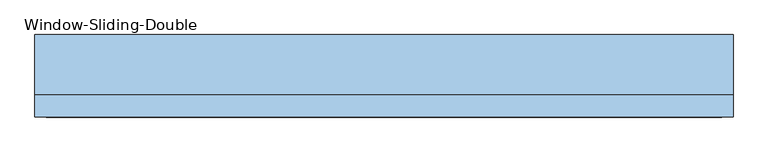
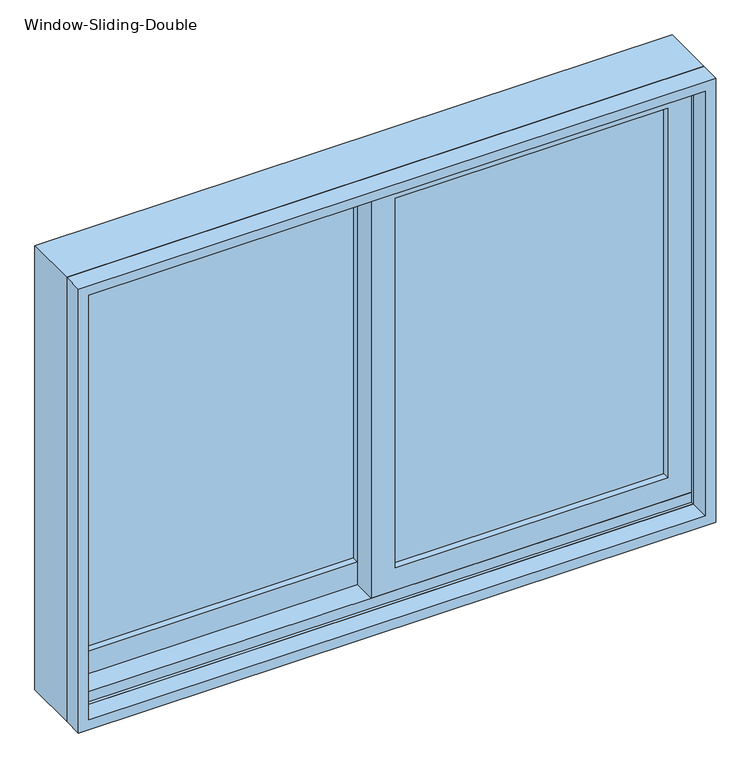
"""IFC4 building model written with IfcOpenShell, lengths in millimetres: window geometry, Window-Sliding-Double."""

from ifc_helpers import new_model, si_unit, frame, origin, place, context, project, spatial, polyline, outline, extrude, faceted_brep, source, transform, mapped, element, save


def window_sliding_double_04af092a(model_context):
    return source(origin(), model_context, "Body", "SolidModel", [
        faceted_brep([(-590.55, -26.035, 914.4), (-590.55, 75.565, 914.4), (590.55, 75.565, 914.4), (590.55, -26.035, 914.4), (-549.6278905, 75.565, 1743.4278905), (-549.6278905, 69.215, 1743.4278905), (-549.6278905, 69.215, 933.45), (-549.6278905, 75.565, 933.45), (549.6278905, 69.215, 1743.4278905), (549.6278905, 69.215, 933.45), (571.5, 69.215, 933.45), (571.5, 69.215, 1765.3), (-571.5, 69.215, 1765.3), (-571.5, 69.215, 933.45), (-571.5, -26.035, 1765.3), (-571.5, -26.035, 933.45), (-571.5, -19.685, 933.45), (-571.5, -19.685, 952.5), (-571.5, 24.765, 952.5), (-571.5, 24.765, 933.45), (590.55, -26.035, 1784.35), (-590.55, -26.035, 1784.35), (571.5, -26.035, 1765.3), (571.5, -26.035, 933.45), (-590.55, 75.565, 1784.35), (590.55, 75.565, 1784.35), (549.6278905, 75.565, 933.45), (549.6278905, 75.565, 1743.4278905), (571.5, 24.765, 933.45), (571.5, 24.765, 952.5), (571.5, -19.685, 952.5), (571.5, -19.685, 933.45)], [[[0, 1, 2, 3]], [[4, 5, 6, 7]], [[5, 8, 9, 10, 11, 12, 13, 6]], [[12, 14, 15, 16, 17, 18, 19, 13]], [[0, 3, 20, 21], [22, 23, 15, 14]], [[24, 1, 0, 21]], [[2, 1, 24, 25], [4, 7, 26, 27]], [[5, 4, 27, 8]], [[12, 11, 22, 14]], [[21, 20, 25, 24]], [[8, 27, 26, 9]], [[22, 11, 10, 28, 29, 30, 31, 23]], [[20, 3, 2, 25]], [[26, 7, 6, 13, 19, 28, 10, 9]], [[28, 19, 18, 29]], [[29, 18, 17, 30]], [[30, 17, 16, 31]], [[15, 23, 31, 16]]]),
        extrude(outline(polyline([(1784.35, -590.55), (914.4, -590.55), (914.4, 590.55), (1784.35, 590.55), (1784.35, -590.55)]), holes=[polyline([(1765.3, 571.5), (933.45, 571.5), (933.45, -571.5), (1765.3, -571.5), (1765.3, 571.5)])]), frame((0.0, -64.135, 0.0), z_axis=(0.0, 1.0, 0.0), x_axis=(0.0, 0.0, 1.0)), (0.0, 0.0, 1.0), 38.1),
        extrude(outline(polyline([(527.05, 12.065), (527.05, 5.715), (22.225, 5.715), (22.225, 12.065), (527.05, 12.065)])), frame((0.0, 0.0, 996.95), z_axis=(0.0, 0.0, 1.0), x_axis=(1.0, 0.0, 0.0)), (0.0, 0.0, 1.0), 723.9),
        extrude(outline(polyline([(527.05, -0.635), (527.05, -6.985), (22.225, -6.985), (22.225, -0.635), (527.05, -0.635)])), frame((0.0, 0.0, 996.95), z_axis=(0.0, 0.0, 1.0), x_axis=(1.0, 0.0, 0.0)), (0.0, 0.0, 1.0), 723.9),
        extrude(outline(polyline([(-22.225, 56.515), (-22.225, 50.165), (-527.05, 50.165), (-527.05, 56.515), (-22.225, 56.515)])), frame((0.0, 0.0, 996.95), z_axis=(0.0, 0.0, 1.0), x_axis=(1.0, 0.0, 0.0)), (0.0, 0.0, 1.0), 723.9),
        extrude(outline(polyline([(-22.225, 43.815), (-22.225, 37.465), (-527.05, 37.465), (-527.05, 43.815), (-22.225, 43.815)])), frame((0.0, 0.0, 996.95), z_axis=(0.0, 0.0, 1.0), x_axis=(1.0, 0.0, 0.0)), (0.0, 0.0, 1.0), 723.9),
        extrude(outline(polyline([(933.45, -571.5), (933.45, 22.225), (1765.3, 22.225), (1765.3, -571.5), (933.45, -571.5)]), holes=[polyline([(1720.85, -22.225), (996.95, -22.225), (996.95, -527.05), (1720.85, -527.05), (1720.85, -22.225)])]), frame((0.0, 24.765, 0.0), z_axis=(0.0, 1.0, 0.0), x_axis=(0.0, 0.0, 1.0)), (0.0, 0.0, 1.0), 44.45),
        extrude(outline(polyline([(952.5, 571.5), (1765.3, 571.5), (1765.3, -22.225), (952.5, -22.225), (952.5, 571.5)]), holes=[polyline([(996.95, 22.225), (1720.85, 22.225), (1720.85, 527.05), (996.95, 527.05), (996.95, 22.225)])]), frame((0.0, -19.685, 0.0), z_axis=(0.0, 1.0, 0.0), x_axis=(0.0, 0.0, 1.0)), (0.0, 0.0, 1.0), 44.45),
    ])


if __name__ == "__main__":
    model = new_model("IFC4")
    model_context = context("Model", 3, world=origin())
    ifc_project = project(units=[si_unit("LENGTHUNIT", "METRE", prefix="MILLI")], contexts=[model_context])
    site = spatial("IfcSite", under=ifc_project)
    building = spatial("IfcBuilding", under=site)
    placement = place(None, origin())
    window_sliding_double_shape = window_sliding_double_04af092a(model_context)
    element("IfcWindow", 1, ObjectType="Window-Sliding-Double : 3' 10 1/2\" x 2'' 10 1/4\"", at=placement, inside=building, context=model_context, shape_type="MappedRepresentation", body=[
        mapped(window_sliding_double_shape, transform((0.0, 0.0, 0.0), x_axis=(1.0, 0.0, 0.0), y_axis=(0.0, 1.0, 0.0), z_axis=(0.0, 0.0, 1.0))),
    ])
    save(model, "model.ifc")

# Revit data of these elements
# Type "Window-Sliding-Double : 3' 10 1/2\" x 2'' 10 1/4\""
#   Type Mark = "22"
#   Fire Rating = "0.5h"
#   Assembly Code = "B2020100"
#   Analytic Construction = "Double glazing - domestic"
#   Window Inset [instance default] = 0' - 0"
#   Wall Thickness [instance default] = 0' - 6"
#   Visual Light Transmittance = 0.81
#   Thermal Resistance (R) = 0.319569 (m²·K)/W
#   Solar Heat Gain Coefficient = 0.76
#   Muntin Width = 1' - 7 7/8"
#   Muntin Height = 2' - 4 1/2"
#   Interior Wall Closure [instance default] = 0' - 2 3/4"
#   Heat Transfer Coefficient (U) = 3.12929 W/(m²·K)
#   Frame Extension [instance default] = 0' - 0 1/4"
#   Exterior Wall Closure [instance default] = 0' - 1 1/4"
#   Rough Width = 3' - 11"
#   Rough Height = 2' - 10 3/4"
#   Height = 2' - 10 1/4"
#   Extension Jamb [instance default] = 0' - 2 3/4"
#   Default Sill Height = 3' - 0"
#   Width = 3' - 10 1/2"
#   Interior Trim Visibility [instance default] = yes
#   Indicator Visibility [instance default] = yes
#   Exterior Trim Visibility [instance default] = yes
#   Muntin Visibility = no
#   Extension Jamb Visibility [instance default] = yes
#   Muntin Pattern = Muntin Pattern_2x2 : Muntin Pattern_2x2
#   Interior Trim Material = Wood - Stained
#   Interior Trim = Trim-Window-Interior-Flat : Picture Frame
#   Interior Frame Material = Wood - Stained
#   Glass Panel Material = Glass
#   Exterior Trim Material = Clad - White
#   Exterior Trim = Trim-Window-Exterior-Flat : with Sill
#   Exterior Frame Material = Clad - White
#   Wall Closure = (empty or 0)
# Element 1 (IfcWindow, "Window-Sliding-Double : 3' 10 1/2\" x 2'' 10 1/4\"")
#   Wall Thickness = 0' - 4 3/4"
#   Extension Jamb = 0' - 1 1/2"
#   Materials on its faces: "Wood - Stained", "Glass", "Clad - White"
# Materials
#   "Wood - Stained": class "Wood", colour RGB 224 178 126, transparency 0, Cost = 0
#   "Glass": class "Glass", colour RGB 236 240 239, transparency 0.85, Description = "Soda Lime Glass", Cost = 0
#   "Clad - White": class "Wood", colour RGB 242 242 238, transparency 0, Cost = 0
